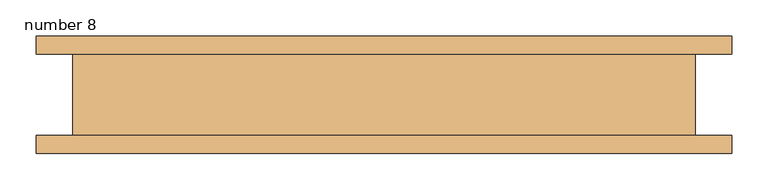
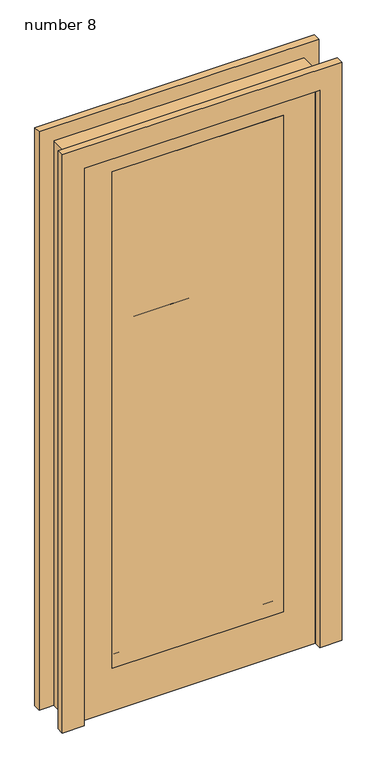
"""IFC4 building model written with IfcOpenShell, lengths in millimetres: door geometry, Doors-Supa_Doors-600_Glass : number 8."""

from ifc_helpers import new_model, si_unit, frame, origin, place, context, project, spatial, polyline, outline, extrude, source, transform, mapped, element, save


def number_8_f6a22701(model_context):
    return source(origin(), model_context, "Body", "SweptSolid", [
        extrude(outline(polyline([(0.0, 431.8000001), (2057.4000001, 431.8000001), (2057.4000001, -431.8000001), (0.0, -431.8000001), (0.0, -406.4000001), (2032.0000001, -406.4000001), (2032.0000001, 406.4000001), (0.0, 406.4000001), (0.0, 431.8000001)])), frame((0.0, -56.35625, 0.0), z_axis=(0.0, 1.0, 0.0), x_axis=(0.0, 0.0, 1.0)), (0.0, 0.0, 1.0), 112.7125),
        extrude(outline(polyline([(0.0, 406.4000001), (2032.0000001, 406.4000001), (2032.0000001, -406.4000001), (0.0, -406.4000001), (0.0, 406.4000001)]), holes=[polyline([(206.375, 31.75), (708.025, 31.75), (708.025, 288.925), (206.375, 288.925), (206.375, 31.75)]), polyline([(1914.5250001, 31.75), (1914.5250001, 288.925), (1412.8750001, 288.925), (1412.8750001, 31.75), (1914.5250001, 31.75)]), polyline([(1412.8750001, -288.925), (1914.5250001, -288.925), (1914.5250001, -31.75), (1412.8750001, -31.75), (1412.8750001, -288.925)]), polyline([(1311.2750001, 31.75), (1311.2750001, 288.925), (809.625, 288.925), (809.625, 31.75), (1311.2750001, 31.75)]), polyline([(809.625, -288.925), (1311.2750001, -288.925), (1311.2750001, -31.75), (809.625, -31.75), (809.625, -288.925)]), polyline([(206.375, -288.925), (708.025, -288.925), (708.025, -31.75), (206.375, -31.75), (206.375, -288.925)])]), frame((0.0, -56.35625, 0.0), z_axis=(0.0, 1.0, 0.0), x_axis=(0.0, 0.0, 1.0)), (0.0, 0.0, 1.0), 44.45),
        extrude(outline(polyline([(2032.0000001, -406.4000001), (2032.0000001, 406.4000001), (0.0, 406.4000001), (0.0, 482.6000001), (2108.2000001, 482.6000001), (2108.2000001, -482.6000001), (0.0, -482.6000001), (0.0, -406.4000001), (2032.0000001, -406.4000001)])), frame((0.0, 56.35625, 0.0), z_axis=(0.0, 1.0, 0.0), x_axis=(0.0, 0.0, 1.0)), (0.0, 0.0, 1.0), 25.4),
        extrude(outline(polyline([(2032.0000001, -406.4000001), (2032.0000001, 406.4000001), (0.0, 406.4000001), (0.0, 482.6000001), (2108.2000001, 482.6000001), (2108.2000001, -482.6000001), (0.0, -482.6000001), (0.0, -406.4000001), (2032.0000001, -406.4000001)])), frame((0.0, -81.75625, 0.0), z_axis=(0.0, 1.0, 0.0), x_axis=(0.0, 0.0, 1.0)), (0.0, 0.0, 1.0), 25.4),
        extrude(outline(polyline([(295.2750001, -57.15), (-295.2750001, -57.15), (-295.2750001, -50.8), (295.2750001, -50.8), (295.2750001, -57.15)])), frame((0.0, 0.0, 155.575), z_axis=(0.0, 0.0, 1.0), x_axis=(1.0, 0.0, 0.0)), (0.0, 0.0, 1.0), 1809.75),
    ])


if __name__ == "__main__":
    model = new_model("IFC4")
    model_context = context("Model", 3, world=origin())
    ifc_project = project(units=[si_unit("LENGTHUNIT", "METRE", prefix="MILLI")], contexts=[model_context])
    site = spatial("IfcSite", under=ifc_project)
    building = spatial("IfcBuilding", under=site)
    placement = place(None, origin())
    number_8_shape = number_8_f6a22701(model_context)
    element("IfcDoor", 1, ObjectType="Doors-Supa_Doors-600_Glass : number 8", at=placement, inside=building, context=model_context, shape_type="MappedRepresentation", body=[
        mapped(number_8_shape, transform((0.0, 0.0, 0.0), x_axis=(1.0, 0.0, 0.0), y_axis=(0.0, 1.0, 0.0), z_axis=(0.0, 0.0, 1.0))),
    ])
    save(model, "model.ifc")

# Revit data of these elements
# Type "Doors-Supa_Doors-600_Glass : number 8"
#   Type Mark = "66"
#   Youtube clip = ""
#   Weight Net (Kg) = "0"
#   Uniclass 2.0 Description = ""
#   Uniclass 2.0 Code = ""
#   Uniclass 1.4 Description = ""
#   Uniclass 1.4 Code = ""
#   URL = "http://supadoor.com/"
#   UNSPSC Name = ""
#   UNSPSC Code = ""
#   Technical description = "http://www.supadoor.com/technical-specifications/3-part-spec.html"
#   Sticking Type = "T"
#   Region South America = "All"
#   Region Oceania = "All"
#   Region North America = "All"
#   Region Middle East = "All"
#   Region Europe = "All"
#   Region Asia = "All"
#   Region Antarctica = "All"
#   Region Africa = "All"
#   QR code = "http://supa-doors.bimobject.com/Glass_Doors_6-Panel"
#   Product group = "Glass Doors"
#   Product family = "Doors"
#   Product data url = "http://supa-doors.bimobject.com/Glass_Doors_6-Panel"
#   Product certification = "http://www.supadoor.com/index.html#"
#   Product SKU = "Glass_Doors_6-Panel"
#   Product Page URL = "http://supadoor.com/standard_doors/panel/general_design.html"
#   Product Name = "600"
#   Product Guid = "b7bd9161-500c-4f3b-9e1f-f23124606a15"
#   Product Documentation Link = "http://supadoor.com/standard_doors/panel/pdf/X-600.pdf"
#   Panel Type = "SC2"
#   Nominal width = "0.00"
#   Nominal height = "0.00"
#   NBS Reference Description = ""
#   NBS Reference Code = ""
#   Model = "600"
#   Material = ""
#   Manufacturer url = "http://supadoor.com/"
#   Manufacturer name = "Supa Doors"
#   Manufacturer country = "United States"
#   Manufacturer = "Supa Doors, Inc."
#   Installation instructions = ""
#   IFC Classification = ""
#   Edition number = "0"
#   EAN code = ""
#   Design country = "United States"
#   Description = "6 Panel Door"
#   Depth = "0.00"
#   Date of publishing = "2014-08-01"
#   COBIe Type Category = ""
#   BIMobject category = ""
#   Analytic Construction = "<None>"
#   Top Rail = 0' - 4 5/8"
#   Thickness = 0' - 1 3/4"
#   Stile Width = 0' - 4 5/8"
#   Rough Width = 2' - 10"
#   Rough Height = 6' - 9"
#   Panel Height = 1' - 7 3/4"
#   Mullion = 0' - 4"
#   Jamb Thickness = 0' - 1"
#   Inset = 0' - 0"
#   Frame Projection Ext. = 0' - 1"
#   Frame Projection Int. = 0' - 1"
#   Frame Width = 0' - 3"
#   Height = 6' - 8"
#   Width = 2' - 8"
#   Center Mullion = 0' - 2 1/2"
#   Bottom Rail = 0' - 8 1/8"
#   Sticking T = yes
#   Sticking S = no
#   Sticking R = no
#   Sticking O = no
#   Sticking E = no
#   Sticking B = no
#   Panel F1 = yes
#   Define Thermal Properties by = 1
#   Door Trim = Wood - Supa Doors - Painted White
#   Door Panel = Wood - Supa Doors - MDF - White
#   Door Glass = Door - Architrave
#   Function = (empty or 0)
#   Wall Closure = (empty or 0)
# Element 1 (IfcDoor, "Doors-Supa_Doors-600_Glass : number 8")
#   Materials on its faces: "Wood - Supa Doors - Painted White", "Wood - Supa Doors - MDF - White", "Door - Architrave"
# Materials
#   "Wood - Supa Doors - Painted White": class "Unassigned", colour RGB 255 255 255, transparency 0
#   "Wood - Supa Doors - MDF - White": class "Unassigned", colour RGB 255 255 255, transparency 0
#   "Door - Architrave": class "Wood", colour RGB 192 192 192, transparency 0, Keynote = "P20", Cost = 0
